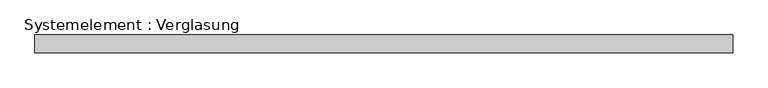
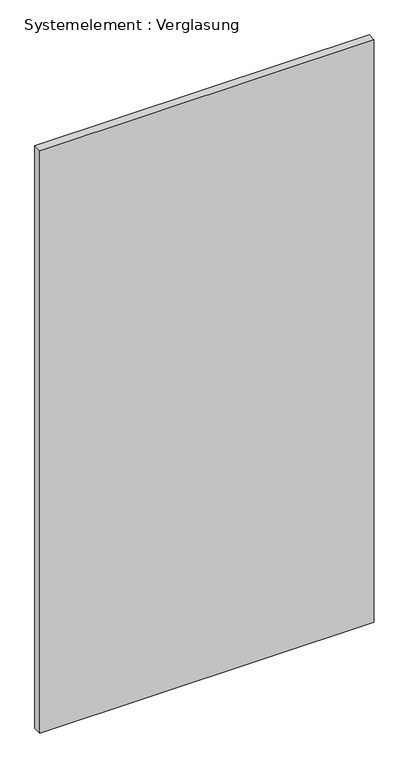
"""IFC4 building model written with IfcOpenShell, lengths in millimetres: plate geometry, Systemelement : Verglasung."""

from ifc_helpers import new_model, si_unit, origin, origin_with_axes, place, context, project, spatial, polyline, outline, extrude, source, transform, mapped, element, save


def systemelement_verglasung_4115e844(model_context):
    return source(origin(), model_context, "Body", "SweptSolid", [
        extrude(outline(polyline([(595.0, -15.0), (-595.0, -15.0), (-595.0, 15.0), (595.0, 15.0), (595.0, -15.0)])), origin_with_axes(), (0.0, 0.0, 1.0), 2190.0),
    ])


if __name__ == "__main__":
    model = new_model("IFC4")
    model_context = context("Model", 3, world=origin())
    ifc_project = project(units=[si_unit("LENGTHUNIT", "METRE", prefix="MILLI")], contexts=[model_context])
    site = spatial("IfcSite", under=ifc_project)
    building = spatial("IfcBuilding", under=site)
    placement = place(None, origin())
    systemelement_verglasung_shape = systemelement_verglasung_4115e844(model_context)
    element("IfcPlate", 1, ObjectType="Systemelement : Verglasung", at=placement, inside=building, context=model_context, shape_type="MappedRepresentation", body=[
        mapped(systemelement_verglasung_shape, transform((0.0, 0.0, 0.0), x_axis=(1.0, 0.0, 0.0), y_axis=(0.0, 1.0, 0.0), z_axis=(0.0, 0.0, 1.0))),
    ])
    save(model, "model.ifc")

# Revit data of these elements
# Type "Systemelement : Verglasung"
#   Construction Type Id = "GSP4R"
#   Analytic Construction = "1/8 Zoll Pilkington-Verglasung einfach"
#   Visual Light Transmittance = 0.9
#   Solar Heat Gain Coefficient = 0.86
#   Heat Transfer Coefficient (U) = 6.7069 W/(m²·K)
# Element 1 (IfcPlate, "Systemelement : Verglasung")
#   Materials on its faces: "Glas"
# Materials
#   "Glas": class "Glas", colour RGB 0 0 255, transparency 0.75, Comments = "Render-Darstellung nicht aktualisiert ", Cost = 0
